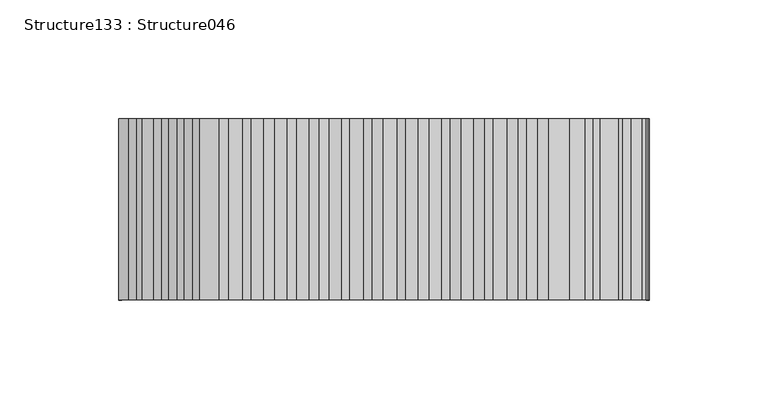
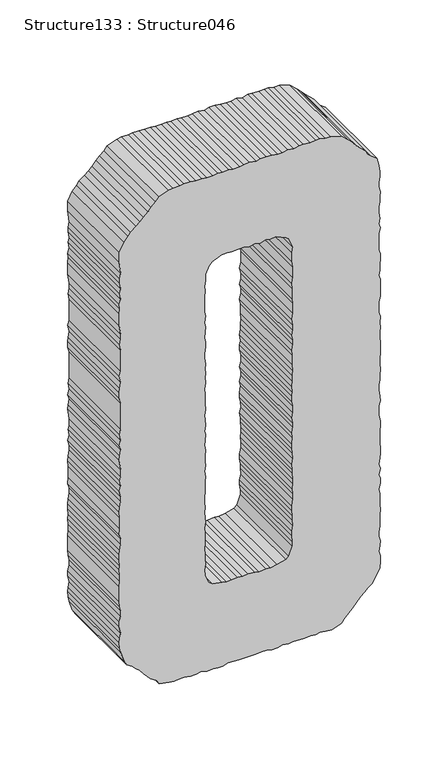
"""IFC4 building model written with IfcOpenShell, lengths in millimetres: proxy geometry, Structure133 : Structure046."""

from ifc_helpers import new_model, si_unit, frame, origin, place, context, project, spatial, polyline, outline, extrude, source, transform, mapped, element, save


def structure133_structure046_99bb57d7(model_context):
    return source(origin(), model_context, "Body", "SweptSolid", [
        extrude(outline(polyline([(3554.0087015, -43068.2737416), (3552.242032, -43059.4933458), (3551.6675836, -43055.3919767), (3552.242032, -43051.2922122), (3552.242032, -43046.6115809), (3551.6675836, -43041.3308275), (3551.6675836, -43036.6501962), (3552.242032, -43032.5488271), (3551.0658569, -43027.2680737), (3551.6675836, -43022.0081802), (3551.0658569, -43017.8843466), (3551.0658569, -43013.7845821), (3552.242032, -43009.1039508), (3552.242032, -43004.4024596), (3551.6675836, -42999.7442928), (3551.6675836, -42985.6590745), (3552.242032, -42980.399181), (3552.242032, -42976.2994165), (3551.0658569, -42971.5963207), (3551.0658569, -42966.917294), (3552.242032, -42962.8159249), (3551.6675836, -42957.5335669), (3552.242032, -42954.0355291), (3551.6675836, -42948.1739089), (3551.6675836, -42944.05168), (3552.242032, -42938.7917864), (3551.6675836, -42934.6904173), (3552.242032, -42930.5906528), (3551.6675836, -42925.9100215), (3551.0658569, -42920.6276635), (3554.0087015, -42912.42653), (3558.1100706, -42909.5077544), (3564.54293, -42903.0444075), (3568.0682461, -42900.1256319), (3572.1423369, -42896.0242628), (3575.0851816, -42892.5037605), (3578.0103756, -42889.5833804), (3580.9532202, -42886.0628781), (3585.6274331, -42883.1424979), (3592.6700423, -42879.6219956), (3597.9540049, -42879.020269), (3603.2122938, -42879.020269), (3607.8961343, -42880.2012579), (3612.5976255, -42879.6219956), (3616.69739, -42879.020269), (3621.3732075, -42880.2012579), (3625.472972, -42880.2012579), (3630.1824862, -42879.6219956), (3640.7167147, -42879.6219956), (3645.4262289, -42879.020269), (3649.5003197, -42879.6219956), (3659.4584952, -42879.6219956), (3663.5598643, -42880.2012579), (3668.8261762, -42879.020269), (3673.5276674, -42879.020269), (3677.0449605, -42880.2012579), (3682.3289231, -42879.020269), (3686.4030139, -42880.2012579), (3691.6869765, -42879.6219956), (3696.3884676, -42879.020269), (3701.0723082, -42879.020269), (3705.1720727, -42879.6219956), (3715.7143242, -42879.6219956), (3720.9726131, -42879.020269), (3725.0996559, -42879.020269), (3730.3563402, -42880.2012579), (3739.1592005, -42880.2012579), (3743.2332913, -42879.020269), (3747.9428055, -42879.6219956), (3753.2171405, -42880.2012579), (3757.8753073, -42880.2012579), (3762.5848215, -42879.6219956), (3767.2590344, -42879.6219956), (3771.3860772, -42879.020269), (3777.2444882, -42879.6219956), (3781.9299333, -42879.6219956), (3786.6298199, -42879.020269), (3795.960595, -42879.020269), (3800.6717138, -42879.6219956), (3805.3459267, -42879.6219956), (3810.0474179, -42879.020269), (3813.5743386, -42879.6219956), (3819.4150989, -42879.020269), (3823.5341187, -42880.2012579), (3832.3161191, -42880.2012579), (3838.1761347, -42879.020269), (3852.8181507, -42879.020269), (3856.9179152, -42880.2012579), (3861.0192843, -42879.6219956), (3866.8776953, -42879.6219956), (3870.4030114, -42879.020269), (3875.686974, -42879.020269), (3879.7610648, -42880.2012579), (3894.4030808, -42880.2012579), (3899.1061766, -42879.020269), (3903.2059411, -42880.2012579), (3907.888177, -42879.6219956), (3913.1641166, -42880.2012579), (3918.4480792, -42880.2012579), (3923.1319197, -42879.6219956), (3927.8077372, -42879.6219956), (3931.9058971, -42879.020269), (3936.6186205, -42880.2012579), (3940.718385, -42880.2012579), (3945.4182716, -42879.6219956), (3950.6765605, -42879.6219956), (3955.9348494, -42880.2012579), (3962.9774586, -42881.961509), (3966.5043792, -42886.6421403), (3969.418341, -42890.1626426), (3973.5197101, -42891.9228937), (3980.5623192, -42899.5239052), (3984.0635662, -42902.4651452), (3987.5792547, -42905.9856475), (3993.4472933, -42912.42653), (3996.390138, -42921.2069258), (3996.390138, -42925.9100215), (3997.5486624, -42930.5906528), (3997.5486624, -42934.1111551), (3996.9645864, -42938.7917864), (3997.5486624, -42944.6534066), (3997.5486624, -42948.1739089), (3996.390138, -42952.8545402), (3997.5486624, -42958.1352936), (3996.390138, -42962.8159249), (3996.390138, -42966.3155673), (3996.9645864, -42971.5963207), (3997.5486624, -42976.2994165), (3997.5486624, -42981.55931), (3996.390138, -42985.0798123), (3997.5486624, -42990.9414325), (3996.9645864, -42995.6204592), (3996.390138, -42999.1425661), (3996.390138, -43005.0041863), (3996.9645864, -43008.5246886), (3996.390138, -43013.7845821), (3996.9645864, -43017.8843466), (3996.390138, -43022.0081802), (3996.390138, -43027.2680737), (3996.9645864, -43031.3678382), (3996.9645864, -43036.6501962), (3997.5486624, -43041.3308275), (3997.5486624, -43046.6115809), (3996.9645864, -43050.1112233), (3996.9645864, -43055.9728435), (3996.390138, -43060.072608), (3993.4472933, -43068.2737416), (3989.9460463, -43071.2165862), (3986.4046842, -43074.7370885), (3983.4794902, -43077.6558641), (3979.3781211, -43081.177971), (3976.4368811, -43084.0967465), (3973.5197101, -43087.6188534), (3969.994394, -43092.2978801), (3967.0788276, -43094.6389981), (3962.9774586, -43098.1595003), (3955.360401, -43102.2608694), (3946.5511223, -43102.2608694), (3936.0345445, -43101.0798805), (3931.3346579, -43101.6816072), (3927.2332888, -43101.6816072), (3921.9733953, -43101.0798805), (3917.8479571, -43101.6816072), (3912.5896682, -43101.0798805), (3908.46423, -43102.2608694), (3904.3901392, -43101.6816072), (3899.7046941, -43102.2608694), (3889.1463965, -43102.2608694), (3880.9452629, -43101.0798805), (3876.263027, -43101.0798805), (3871.5599312, -43101.6816072), (3866.3032469, -43101.0798805), (3847.5598618, -43101.0798805), (3843.432819, -43102.2608694), (3837.6000817, -43101.0798805), (3832.3161191, -43101.6816072), (3828.790803, -43102.2608694), (3823.5341187, -43102.2608694), (3818.8310229, -43101.0798805), (3795.4037973, -43101.0798805), (3790.7039107, -43101.6816072), (3785.4456218, -43101.0798805), (3780.7441306, -43102.2608694), (3776.6427615, -43101.0798805), (3771.3860772, -43101.6816072), (3767.8607611, -43102.2608694), (3758.485057, -43101.0798805), (3752.6170184, -43101.0798805), (3749.117376, -43101.6816072), (3743.8414364, -43101.0798805), (3739.7416719, -43102.2608694), (3734.47536, -43101.0798805), (3730.3563402, -43101.0798805), (3725.0996559, -43101.6816072), (3720.9726131, -43102.2608694), (3715.7143242, -43101.6816072), (3705.7545441, -43101.6816072), (3700.4705815, -43102.2608694), (3696.3884676, -43101.0798805), (3691.6869765, -43101.0798805), (3686.4030139, -43101.6816072), (3682.3289231, -43102.2608694), (3677.6274319, -43102.2608694), (3672.3691429, -43101.6816072), (3668.8261762, -43102.2608694), (3663.5598643, -43101.6816072), (3658.3015753, -43101.6816072), (3653.6000842, -43102.2608694), (3640.114988, -43102.2608694), (3635.4407751, -43101.6816072), (3631.3410106, -43101.0798805), (3626.6571701, -43101.0798805), (3621.9813526, -43102.2608694), (3617.2718384, -43102.2608694), (3611.4134274, -43101.0798805), (3606.7295868, -43101.6816072), (3603.2122938, -43102.2608694), (3597.9540049, -43101.6816072), (3593.8285667, -43101.0798805), (3585.0706354, -43098.1595003), (3580.9532202, -43095.819987), (3578.0103756, -43091.1393557), (3574.5107332, -43087.6188534), (3572.1423369, -43084.6984732), (3567.4857747, -43081.177971), (3561.025637, -43075.3163507), (3558.1100706, -43070.6357194), (3554.0087015, -43068.2737416)]), holes=[polyline([(3918.4480792, -42959.8746849), (3916.6653636, -42957.5335669), (3908.46423, -42954.0355291), (3903.7884125, -42955.1940536), (3895.5888836, -42955.1940536), (3890.320967, -42954.0355291), (3880.9452629, -42954.0355291), (3875.686974, -42955.1940536), (3870.9790644, -42954.6147914), (3861.6178018, -42954.6147914), (3858.1021133, -42954.0355291), (3848.7167816, -42954.0355291), (3843.432819, -42955.1940536), (3838.1761347, -42954.0355291), (3833.4730389, -42954.0355291), (3828.790803, -42955.1940536), (3824.7167122, -42954.0355291), (3820.5896694, -42954.0355291), (3815.3313805, -42955.1940536), (3811.2043377, -42954.6147914), (3802.448011, -42954.6147914), (3797.1463977, -42954.0355291), (3792.4705802, -42954.6147914), (3787.7867397, -42954.6147914), (3783.0868532, -42955.1940536), (3777.8285642, -42954.6147914), (3774.3032481, -42955.1940536), (3769.6274306, -42955.1940536), (3764.9435901, -42954.0355291), (3759.0595054, -42954.0355291), (3754.3756649, -42955.1940536), (3749.701452, -42954.0355291), (3746.1745313, -42954.0355291), (3740.9162424, -42955.1940536), (3736.7988273, -42954.6147914), (3730.9323932, -42955.1940536), (3726.8566978, -42955.1940536), (3722.7312597, -42954.6147914), (3717.4729707, -42954.0355291), (3712.7971532, -42955.1940536), (3708.087639, -42954.6147914), (3704.5879966, -42954.6147914), (3699.3136616, -42954.0355291), (3695.2122926, -42954.0355291), (3690.512406, -42954.6147914), (3685.8285655, -42954.0355291), (3681.1447249, -42954.0355291), (3675.2863139, -42955.1940536), (3671.1849448, -42955.1940536), (3666.5027089, -42954.6147914), (3662.3836892, -42954.6147914), (3657.1254002, -42954.0355291), (3652.4431643, -42955.1940536), (3648.3161216, -42955.1940536), (3643.0578326, -42954.6147914), (3638.9580681, -42954.6147914), (3630.7392839, -42957.5335669), (3628.4158166, -42959.8746849), (3626.6571701, -42967.4965562), (3625.472972, -42972.7773096), (3626.0554434, -42976.8786787), (3625.472972, -42982.740299), (3626.0554434, -42986.2608012), (3626.6571701, -42992.1224214), (3626.0554434, -42996.8030528), (3626.6571701, -43000.9028172), (3626.0554434, -43006.1851752), (3626.0554434, -43010.2849397), (3626.6571701, -43014.3863088), (3628.4158166, -43022.5649779), (3630.7392839, -43025.506218), (3637.7995437, -43028.4490626), (3643.0578326, -43029.0283248), (3648.3161216, -43027.8473359), (3651.8590883, -43028.4490626), (3657.1254002, -43028.4490626), (3662.3836892, -43029.0283248), (3667.0851803, -43028.4490626), (3675.8687854, -43028.4490626), (3681.1447249, -43029.0283248), (3685.8285655, -43027.8473359), (3689.9540036, -43028.4490626), (3694.6298211, -43029.0283248), (3699.8881101, -43028.4490626), (3703.4134261, -43029.0283248), (3708.6717151, -43029.0283248), (3713.3555556, -43028.4490626), (3723.3313817, -43028.4490626), (3726.8566978, -43027.8473359), (3732.1149867, -43029.0283248), (3736.7988273, -43027.8473359), (3740.3161203, -43028.4490626), (3746.1745313, -43028.4490626), (3750.8583719, -43027.8473359), (3755.559863, -43029.0283248), (3759.6596275, -43028.4490626), (3764.9435901, -43027.8473359), (3768.4432325, -43029.0283248), (3773.11905, -43027.8473359), (3782.5027771, -43029.0283248), (3787.7867397, -43027.8473359), (3792.4705802, -43028.4490626), (3801.2718359, -43028.4490626), (3806.5317294, -43029.0283248), (3811.7884138, -43027.8473359), (3816.4883003, -43028.4490626), (3820.5896694, -43027.8473359), (3824.1149855, -43028.4490626), (3828.790803, -43027.8473359), (3834.0474873, -43029.0283248), (3838.1761347, -43029.0283248), (3844.0345457, -43027.8473359), (3848.1166595, -43027.8473359), (3852.2340747, -43029.0283248), (3858.1021133, -43028.4490626), (3861.6178018, -43027.8473359), (3866.3032469, -43029.0283248), (3872.1440073, -43027.8473359), (3875.686974, -43029.0283248), (3889.7208449, -43029.0283248), (3895.0048075, -43028.4490626), (3899.1061766, -43029.0283248), (3903.7884125, -43027.8473359), (3909.6468235, -43027.8473359), (3916.0909152, -43024.9269558), (3919.0321552, -43022.5649779), (3922.5494483, -43014.3863088), (3922.5494483, -43009.683213), (3921.9733953, -43005.5834486), (3922.5494483, -43000.3010906), (3922.5494483, -42995.6204592), (3921.3748778, -42990.9414325), (3922.5494483, -42986.2608012), (3921.3748778, -42981.55931), (3922.5494483, -42976.8786787), (3921.9733953, -42972.7773096), (3922.5494483, -42968.0982829), (3918.4480792, -42959.8746849)])]), frame((0.0, 247945.1599557, 0.0), z_axis=(0.0, 1.0, 0.0), x_axis=(0.0, 0.0, 1.0)), (0.0, 0.0, 1.0), 76.2),
    ])


if __name__ == "__main__":
    model = new_model("IFC4")
    model_context = context("Model", 3, world=origin())
    ifc_project = project(units=[si_unit("LENGTHUNIT", "METRE", prefix="MILLI")], contexts=[model_context])
    site = spatial("IfcSite", under=ifc_project)
    building = spatial("IfcBuilding", under=site)
    placement = place(None, origin())
    structure133_structure046_shape = structure133_structure046_99bb57d7(model_context)
    element("IfcBuildingElementProxy", 1, Name="Structure133 : Structure046", ObjectType="Structure133 : Structure046", at=placement, inside=building, context=model_context, shape_type="MappedRepresentation", body=[
        mapped(structure133_structure046_shape, transform((0.0, 0.0, 0.0), x_axis=(1.0, 0.0, 0.0), y_axis=(0.0, 1.0, 0.0), z_axis=(0.0, 0.0, 1.0))),
    ])
    save(model, "model.ifc")

# Revit data of these elements
# Type "Structure133 : Structure046"
#   NameOverride = "Structure046"
# Element 1 (IfcBuildingElementProxy, "Structure133 : Structure046")
#   Materials on its faces: "BRUSHED ALUM. LETTERING"
# Materials
#   "BRUSHED ALUM. LETTERING": class "Unassigned", colour RGB 169 181 186, transparency 0, Cost = 0
